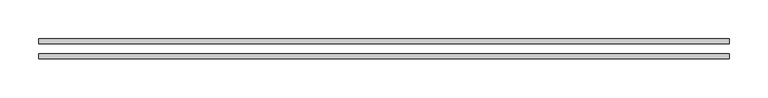
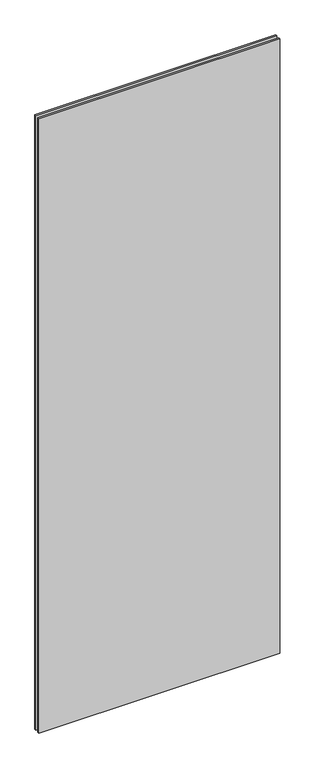
"""IFC4 building model written with IfcOpenShell, lengths in millimetres: proxy geometry, Window glass:Window glass:300352:Window glass:300352 : Window glass:Window glass:300352:300073:Window glass:300352:Window glass:300352 : Window glass:Window glass:300352:300073 : Window glass:Window glass:300352:Window glass:300352 : Window glass:Window glass:300352:300073:3 : Window glass:Window glass:300352:Window glass:300352 : Window glass:Window glass:300352:300073:Window glass:300352:Window glass:300352 : Window glass:Window glass:300352:300073 : Window glass:Window glass:300352:Window glass:300352 : Window glass:Window glass:300352:300073:300061."""

from ifc_helpers import new_model, si_unit, frame, origin, place, context, project, spatial, polyline, outline, extrude, source, transform, mapped, element, save


def generic_models_7430f0a1(model_context):
    return source(origin(), model_context, "Body", "SweptSolid", [
        extrude(outline(polyline([(570404.7161787, -579048.3332724), (569517.8947692, -579048.3332724), (569517.8947692, -579041.9832724), (570404.7161787, -579041.9832724), (570404.7161787, -579048.3332724)])), frame((0.0, 0.0, 55.1405965), z_axis=(0.0, 0.0, 1.0), x_axis=(1.0, 0.0, 0.0)), (0.0, 0.0, 1.0), 2392.531079),
        extrude(outline(polyline([(570404.7161787, -579029.2832724), (569517.8947692, -579029.2832724), (569517.8947692, -579022.9332724), (570404.7161787, -579022.9332724), (570404.7161787, -579029.2832724)])), frame((0.0, 0.0, 55.1405965), z_axis=(0.0, 0.0, 1.0), x_axis=(1.0, 0.0, 0.0)), (0.0, 0.0, 1.0), 2392.531079),
    ])


if __name__ == "__main__":
    model = new_model("IFC4")
    model_context = context("Model", 3, world=origin())
    ifc_project = project(units=[si_unit("LENGTHUNIT", "METRE", prefix="MILLI")], contexts=[model_context])
    site = spatial("IfcSite", under=ifc_project)
    building = spatial("IfcBuilding", under=site)
    placement = place(None, origin())
    generic_models_shape = generic_models_7430f0a1(model_context)
    element("IfcBuildingElementProxy", 1, Name="Window glass:Window glass:300352:Window glass:300352 : Window glass:Window glass:300352:300073:Window glass:300352:Window glass:300352 : Window glass:Window glass:300352:300073 : Window glass:Window glass:300352:Window glass:300352 : Window glass:Window glass:300352:300073:3 : Window glass:Window glass:300352:Window glass:300352 : Window glass:Window glass:300352:300073:Window glass:300352:Window glass:300352 : Window glass:Window glass:300352:300073 : Window glass:Window glass:300352:Window glass:300352 : Window glass:Window glass:300352:300073:300061", ObjectType="Window glass:Window glass:300352:Window glass:300352 : Window glass:Window glass:300352:300073:Window glass:300352:Window glass:300352 : Window glass:Window glass:300352:300073 : Window glass:Window glass:300352:Window glass:300352 : Window glass:Window glass:300352:300073:3 : Window glass:Window glass:300352:Window glass:300352 : Window glass:Window glass:300352:300073:Window glass:300352:Window glass:300352 : Window glass:Window glass:300352:300073 : Window glass:Window glass:300352:Window glass:300352 : Window glass:Window glass:300352:300073:300061", at=placement, inside=building, context=model_context, shape_type="MappedRepresentation", body=[
        mapped(generic_models_shape, transform((0.0, 0.0, 0.0), x_axis=(1.0, 0.0, 0.0), y_axis=(0.0, 1.0, 0.0), z_axis=(0.0, 0.0, 1.0))),
    ])
    save(model, "model.ifc")

# Revit data of these elements
# Type "Window glass:Window glass:300352:Window glass:300352 : Window glass:Window glass:300352:300073:Window glass:300352:Window glass:300352 : Window glass:Window glass:300352:300073 : Window glass:Window glass:300352:Window glass:300352 : Window glass:Window glass:300352:300073:3 : Window glass:Window glass:300352:Window glass:300352 : Window glass:Window glass:300352:300073:Window glass:300352:Window glass:300352 : Window glass:Window glass:300352:300073 : Window glass:Window glass:300352:Window glass:300352 : Window glass:Window glass:300352:300073:300061"
#   NameOverride = "Window glass:Window glass:300352:Window glass:300352 : Window glass:Window glass:300352:300073:Window glass:300352:Window glass:300352 : Window glass:Window glass:300352:300073 : Window glass:Window glass:300352:Window glass:300352 : Window glass:Window glass:300352:300073:300061"
#   ObjectTypeOverride = "Window glass:300352:Window glass:300352 : Window glass:Window glass:300352:300073 : Window glass:Window glass:300352:Window glass:300352 : Window glass:Window glass:300352:300073"
#   Reference = "Window glass"
#   Tag = "300061"
# Element 1 (IfcBuildingElementProxy, "Window glass:Window glass:300352:Window glass:300352 : Window glass:Window glass:300352:300073:Window glass:300352:Window glass:300352 : Window glass:Window glass:300352:300073 : Window glass:Window glass:300352:Window glass:300352 : Window glass:Window glass:300352:300073:3 : Window glass:Window glass:300352:Window glass:300352 : Window glass:Window glass:300352:300073:Window glass:300352:Window glass:300352 : Window glass:Window glass:300352:300073 : Window glass:Window glass:300352:Window glass:300352 : Window glass:Window glass:300352:300073:300061")
#   Materials on its faces: "INSULATED LOW-E GLAZING (SEE ELEVATIONS FOR U-FACTOR, SHGC, & LT)"
# Materials
#   "INSULATED LOW-E GLAZING (SEE ELEVATIONS FOR U-FACTOR, SHGC, & LT)": class "Unassigned", colour RGB 84 171 255, transparency 0, Cost = 0
